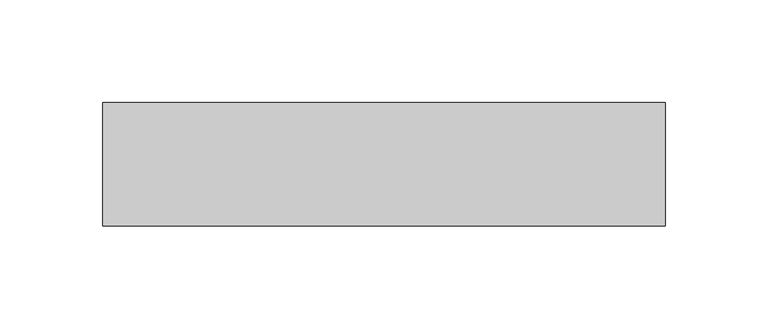
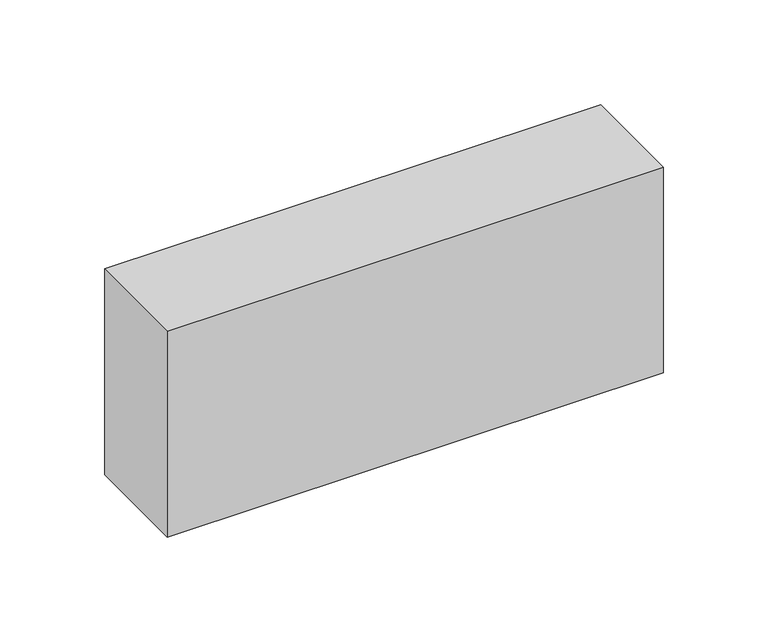
"""IFC4 building model written with IfcOpenShell, lengths in millimetres: beam geometry, Madeira de lei : Berço 6x12cm."""

from ifc_helpers import new_model, si_unit, frame, origin, place, context, project, spatial, polyline, outline, extrude, source, transform, mapped, element, save


def beam_88f0ebe1(model_context):
    return source(origin(), model_context, "Body", "SweptSolid", [
        extrude(outline(polyline([(136.7503096, 30.0), (136.7503096, -30.0), (-136.7503096, -30.0), (-136.7503096, 30.0), (136.7503096, 30.0)])), frame((0.0, 0.0, -60.0), z_axis=(0.0, 0.0, 1.0), x_axis=(1.0, 0.0, 0.0)), (0.0, 0.0, 1.0), 120.0),
    ])


if __name__ == "__main__":
    model = new_model("IFC4")
    model_context = context("Model", 3, world=origin())
    ifc_project = project(units=[si_unit("LENGTHUNIT", "METRE", prefix="MILLI")], contexts=[model_context])
    site = spatial("IfcSite", under=ifc_project)
    building = spatial("IfcBuilding", under=site)
    placement = place(None, origin())
    beam_shape = beam_88f0ebe1(model_context)
    element("IfcBeam", 1, ObjectType="Madeira de lei : Berço 6x12cm", at=placement, inside=building, context=model_context, shape_type="MappedRepresentation", body=[
        mapped(beam_shape, transform((0.0, 0.0, 0.0), x_axis=(1.0, 0.0, 0.0), y_axis=(0.0, 1.0, 0.0), z_axis=(0.0, 0.0, 1.0))),
    ])
    save(model, "model.ifc")

# Revit data of these elements
# Type "Madeira de lei : Berço 6x12cm"
#   A = 0.02 m²
#   Length [instance default] = 1.524 m
#   b = 0.06 m
#   d = 0.12 m
#   Structural Material [instance default] = none
#   Assembly Code = ""
# Element 1 (IfcBeam, "Madeira de lei : Berço 6x12cm")
#   Structural Material = .MADEIRAMENTO
#   Materials on its faces: ".MADEIRAMENTO"
# Materials
#   ".MADEIRAMENTO": class ".CC_MADEIRAS", colour RGB 212 179 113, transparency 0, Cost = 0
